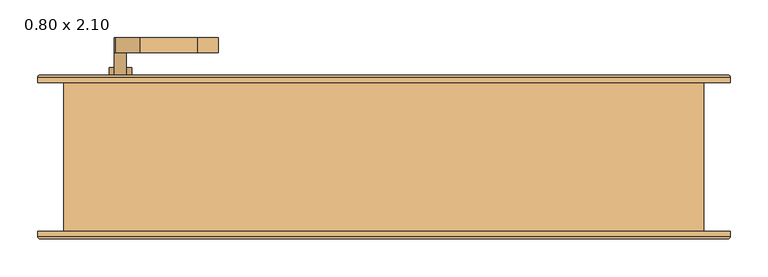
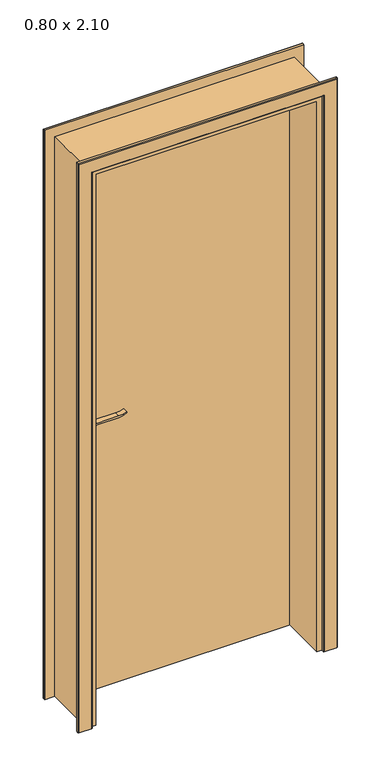
"""IFC4 building model written with IfcOpenShell, lengths in millimetres: door geometry, .CC_ND 300_PORTA SIMPLES DE ABRIR_COM EXTENSÃO : 0.80 x 2.10."""

import ifcopenshell
import ifcopenshell.guid

model = None  # the IFC model being written
_history = None  # IfcOwnerHistory: only IFC2X3 demands one
_inside = {}  # id of a spatial element -> (the spatial element, [elements in it])
_under = {}  # id of a project, library or spatial element -> (it, [spatial elements below it])
_declared = {}  # id of a project -> (the project, [libraries it declares])
_typed = {}  # id of a type object -> (the type object, [elements of that type])
_made_of = {}  # id of a material, layer set ... -> (it, [elements and type objects made of it])


def new_model(schema):
    """Start an empty IFC model of exactly this schema.

    Asked for "IFC4X3", IfcOpenShell would pick the latest addendum, in which some entities
    have other attributes; the version numbers below select the first issue.
    IFC2X3 requires an IfcOwnerHistory on every rooted entity: one is made here for all.
    """
    global model, _history
    if schema == "IFC4X3":
        model = ifcopenshell.file(schema_version=(4, 3, 0, 0))
    else:
        model = ifcopenshell.file(schema=schema)
    _inside.clear()
    _under.clear()
    _declared.clear()
    _typed.clear()
    _made_of.clear()
    _history = None
    if model.schema == "IFC2X3":
        org = make("IfcOrganization", Name="unknown")
        user = make(
            "IfcPersonAndOrganization",
            ThePerson=make("IfcPerson", FamilyName="unknown"),
            TheOrganization=org,
        )
        app = make(
            "IfcApplication",
            ApplicationDeveloper=org,
            Version="unknown",
            ApplicationFullName="unknown",
            ApplicationIdentifier="unknown",
        )
        _history = make(
            "IfcOwnerHistory",
            OwningUser=user,
            OwningApplication=app,
            ChangeAction="ADDED",
            CreationDate=0,
        )
    return model


def make(cls, **values):
    """One entity of the class cls with the attributes given. An attribute that is None is left unset."""
    return model.create_entity(
        cls, **{name: value for name, value in values.items() if value is not None}
    )


def rooted(cls, **values):
    """An entity with a GlobalId (a new one), such as an element, a storey or a relation."""
    return make(cls, GlobalId=ifcopenshell.guid.new(), OwnerHistory=_history, **values)


def si_unit(unit_type, name, prefix=None):
    """IfcSIUnit, for example si_unit("LENGTHUNIT", "METRE", prefix="MILLI")."""
    return make("IfcSIUnit", UnitType=unit_type, Prefix=prefix, Name=name)


def assignment(units):
    """IfcUnitAssignment: the units of a project."""
    return None if units is None else make("IfcUnitAssignment", Units=units)


def point(xyz):
    """IfcCartesianPoint."""
    return None if xyz is None else make("IfcCartesianPoint", Coordinates=xyz)


def direction(xyz):
    """IfcDirection."""
    return None if xyz is None else make("IfcDirection", DirectionRatios=xyz)


def frame(location, z_axis=None, x_axis=None):
    """IfcAxis2Placement3D, a coordinate frame: its origin and axes. An axis left out is left unset."""
    return make(
        "IfcAxis2Placement3D",
        Location=point(location),
        Axis=direction(z_axis),
        RefDirection=direction(x_axis),
    )


def frame_2d(location, x_axis=None):
    """IfcAxis2Placement2D, a coordinate frame in the plane: its origin and x axis."""
    return make(
        "IfcAxis2Placement2D", Location=point(location), RefDirection=direction(x_axis)
    )


def origin():
    """The frame at (0, 0, 0) with its axes left unset."""
    return frame((0.0, 0.0, 0.0))


def origin_with_axes():
    """The frame at (0, 0, 0) with the z axis (0, 0, 1) and the x axis (1, 0, 0) written out."""
    return frame((0.0, 0.0, 0.0), z_axis=(0.0, 0.0, 1.0), x_axis=(1.0, 0.0, 0.0))


def place(relative_to, where):
    """IfcLocalPlacement: puts the frame where relative to a parent placement (None: the world)."""
    return make(
        "IfcLocalPlacement", PlacementRelTo=relative_to, RelativePlacement=where
    )


def context(
    kind, dimensions, precision=None, world=None, true_north=None, identifier=None
):
    """IfcGeometricRepresentationContext, for example the 3D "Model" context."""
    return make(
        "IfcGeometricRepresentationContext",
        ContextIdentifier=identifier,
        ContextType=kind,
        CoordinateSpaceDimension=dimensions,
        Precision=precision,
        WorldCoordinateSystem=world,
        TrueNorth=true_north,
    )


def project(units=None, contexts=None):
    """IfcProject with its units and contexts."""
    return rooted(
        "IfcProject",
        Name="project",
        RepresentationContexts=contexts,
        UnitsInContext=assignment(units),
    )


def spatial(cls, under=None, at=None, **own):
    """A site, building, storey or space (cls), placed at a placement, below another one or the project."""
    s = rooted(cls, ObjectPlacement=at, **own)
    if under is not None:
        _under.setdefault(under.id(), (under, []))[1].append(s)
    return s


def polyline(points):
    """IfcPolyline through the points."""
    return make("IfcPolyline", Points=[point(p) for p in points])


def circle_curve(where, radius):
    """IfcCircle in the frame where."""
    return make("IfcCircle", Position=where, Radius=radius)


def ellipse_curve(where, semi_axis1, semi_axis2):
    """IfcEllipse in the frame where."""
    return make(
        "IfcEllipse", Position=where, SemiAxis1=semi_axis1, SemiAxis2=semi_axis2
    )


def trimmed(basis, trim1, trim2, sense, master):
    """IfcTrimmedCurve: the piece of a basis curve between two trims."""
    return make(
        "IfcTrimmedCurve",
        BasisCurve=basis,
        Trim1=trim1,
        Trim2=trim2,
        SenseAgreement=sense,
        MasterRepresentation=master,
    )


def segment(curve, same_sense, transition):
    """IfcCompositeCurveSegment."""
    return make(
        "IfcCompositeCurveSegment",
        Transition=transition,
        SameSense=same_sense,
        ParentCurve=curve,
    )


def composite_curve(segments, self_intersect=None):
    """IfcCompositeCurve: segments joined end to end."""
    return make("IfcCompositeCurve", Segments=segments, SelfIntersect=self_intersect)


def outline(outer, holes=None, kind="AREA"):
    """IfcArbitraryClosedProfileDef: a profile drawn as a closed curve; with holes, ...WithVoids."""
    if holes is None:
        return make("IfcArbitraryClosedProfileDef", ProfileType=kind, OuterCurve=outer)
    return make(
        "IfcArbitraryProfileDefWithVoids",
        ProfileType=kind,
        OuterCurve=outer,
        InnerCurves=holes,
    )


def extrude(swept, where, along, depth):
    """IfcExtrudedAreaSolid: the profile swept, set in the frame where, extruded along a direction by depth."""
    return make(
        "IfcExtrudedAreaSolid",
        SweptArea=swept,
        Position=where,
        ExtrudedDirection=direction(along),
        Depth=depth,
    )


def faces_of(points, faces, orient=None, outer=None):
    """IfcFace entities. A face is a list of loops; a loop is a list of indices into points, from 0.

    orient and outer hold one flag for each loop. By default every Orientation is true, the
    first loop of a face is its IfcFaceOuterBound and the others are IfcFaceBound.
    """
    made = []
    for i, loops in enumerate(faces):
        bounds = []
        for j, loop in enumerate(loops):
            is_outer = j == 0 if outer is None else outer[i][j]
            bounds.append(
                make(
                    "IfcFaceOuterBound" if is_outer else "IfcFaceBound",
                    Bound=make("IfcPolyLoop", Polygon=[points[k] for k in loop]),
                    Orientation=True if orient is None else orient[i][j],
                )
            )
        made.append(make("IfcFace", Bounds=bounds))
    return made


def faceted_brep(points, faces, orient=None, outer=None, voids=None):
    """IfcFacetedBrep: a solid bounded by flat faces; with voids (closed shells), ...WithVoids."""
    shared = [point(p) for p in points]
    hull = make("IfcClosedShell", CfsFaces=faces_of(shared, faces, orient, outer))
    if voids is None:
        return make("IfcFacetedBrep", Outer=hull)
    return make(
        "IfcFacetedBrepWithVoids",
        Outer=hull,
        Voids=[
            make(cls, CfsFaces=faces_of(shared, fs, o, b)) for cls, fs, o, b in voids
        ],
    )


def shape(context_of_items, identifier, shape_type, items):
    """IfcShapeRepresentation: the items that make up one representation, for example the "Body"."""
    return make(
        "IfcShapeRepresentation",
        ContextOfItems=context_of_items,
        RepresentationIdentifier=identifier,
        RepresentationType=shape_type,
        Items=items,
    )


def source(mapping_origin, context_of_items, identifier, shape_type, items):
    """IfcRepresentationMap: a shape defined once, which mapped items show again and again."""
    return make(
        "IfcRepresentationMap",
        MappingOrigin=mapping_origin,
        MappedRepresentation=shape(context_of_items, identifier, shape_type, items),
    )


def transform(
    local_origin,
    x_axis=None,
    y_axis=None,
    z_axis=None,
    scale=None,
    scale2=None,
    scale3=None,
    uniform=True,
):
    """IfcCartesianTransformationOperator3D, or its non-uniform kind. x_axis, y_axis, z_axis: its Axis1, 2, 3."""
    if uniform:
        return make(
            "IfcCartesianTransformationOperator3D",
            Axis1=direction(x_axis),
            Axis2=direction(y_axis),
            LocalOrigin=point(local_origin),
            Scale=scale,
            Axis3=direction(z_axis),
        )
    return make(
        "IfcCartesianTransformationOperator3DnonUniform",
        Axis1=direction(x_axis),
        Axis2=direction(y_axis),
        LocalOrigin=point(local_origin),
        Scale=scale,
        Axis3=direction(z_axis),
        Scale2=scale2,
        Scale3=scale3,
    )


def mapped(mapping_source, mapping_target):
    """IfcMappedItem: shows the shape of a source again, moved by a transform."""
    return make(
        "IfcMappedItem", MappingSource=mapping_source, MappingTarget=mapping_target
    )


def made_of(thing, what):
    """Note that an element or type object is made of a material, layer set ...; save() writes the relation."""
    if what is not None:
        _made_of.setdefault(what.id(), (what, []))[1].append(thing)
    return thing


def element(
    cls,
    number,
    at=None,
    inside=None,
    cuts=None,
    type_object=None,
    material=None,
    context=None,
    identifier="Body",
    shape_type=None,
    held_by="IfcProductDefinitionShape",
    body=None,
    shapes=None,
    **own,
):
    """One element of the class cls, such as IfcWall. Its Tag is "e" and its number.

    at: its placement. inside: the storey or other place that contains it. cuts: it is an
    opening in that element (IfcRelVoidsElement). A single representation is given by context,
    identifier, shape_type and body (its items); several are given by shapes. held_by: the class
    of the entity that holds the representations. save() writes the other relations.
    """
    e = rooted(cls, Tag="e%d" % number, ObjectPlacement=at, **own)
    if body is not None:
        shapes = [shape(context, identifier, shape_type, body)]
    if shapes is not None:
        e.Representation = make(held_by, Representations=shapes)
    if inside is not None:
        _inside.setdefault(inside.id(), (inside, []))[1].append(e)
    if cuts is not None:
        rooted(
            "IfcRelVoidsElement", RelatingBuildingElement=cuts, RelatedOpeningElement=e
        )
    if type_object is not None:
        _typed.setdefault(type_object.id(), (type_object, []))[1].append(e)
    return made_of(e, material)


def aggregate(whole, parts):
    """IfcRelAggregates: a whole, such as a stair, and the parts it consists of."""
    return rooted("IfcRelAggregates", RelatingObject=whole, RelatedObjects=parts)


def save(model, path):
    """Write the relations noted so far, then the file.

    IfcRelAggregates (storeys below a building ...), IfcRelContainedInSpatialStructure (elements
    in a storey), IfcRelDefinesByType, IfcRelAssociatesMaterial and IfcRelDeclares: one each for
    every whole, place, type object, material and project.
    """
    for whole, parts in _under.values():
        aggregate(whole, parts)
    for where, things in _inside.values():
        rooted(
            "IfcRelContainedInSpatialStructure",
            RelatedElements=things,
            RelatingStructure=where,
        )
    for kind, things in _typed.values():
        rooted("IfcRelDefinesByType", RelatedObjects=things, RelatingType=kind)
    for what, things in _made_of.values():
        rooted("IfcRelAssociatesMaterial", RelatedObjects=things, RelatingMaterial=what)
    for by, libraries in _declared.values():
        rooted("IfcRelDeclares", RelatingContext=by, RelatedDefinitions=libraries)
    model.write(path)


def plane_surface(at):
    """IfcPlane: the flat surface through the origin of the frame at, square to its z axis."""
    return make("IfcPlane", Position=at)


def cylinder_surface(at, radius):
    """IfcCylindricalSurface: all points at the distance radius from the z axis of the frame at."""
    return make("IfcCylindricalSurface", Position=at, Radius=radius)


def advanced_brep(points, edges, surfaces, faces):
    """IfcAdvancedBrep: a solid bounded by faces that lie on surfaces and meet in shared edges.

    An edge is (start, end): straight between two places in points (the first is 0);
    or (start, end, curve); or (start, end, curve, False) where it runs against its curve.
    A face is (place in surfaces, loops), or (place, loops, False) where it looks against
    its surface's normal. A loop lists edges by number (the first is 1), with a minus sign
    where the edge is run from its end to its start. The first loop is the outer one.
    """
    corners = [point(p) for p in points]
    vertices = [make("IfcVertexPoint", VertexGeometry=c) for c in corners]
    made = []
    for start, end, *more in edges:
        made.append(
            make(
                "IfcEdgeCurve",
                EdgeStart=vertices[start],
                EdgeEnd=vertices[end],
                EdgeGeometry=more[0] if more else make("IfcPolyline", Points=[corners[start], corners[end]]),
                SameSense=more[1] if len(more) > 1 else True,
            )
        )
    hull = []
    for where, loops, *sense in faces:
        bounds = []
        for j, loop in enumerate(loops):
            ring = [make("IfcOrientedEdge", EdgeElement=made[abs(k) - 1], Orientation=k > 0) for k in loop]
            bounds.append(
                make(
                    "IfcFaceOuterBound" if j == 0 else "IfcFaceBound",
                    Bound=make("IfcEdgeLoop", EdgeList=ring),
                    Orientation=True,
                )
            )
        hull.append(make("IfcAdvancedFace", Bounds=bounds, FaceSurface=surfaces[where], SameSense=sense[0] if sense else True))
    return make("IfcAdvancedBrep", Outer=make("IfcClosedShell", CfsFaces=hull))


def door_0_80_x_2_10_6188e507(model_context):
    return source(origin(), model_context, "Body", "SolidModel", [
        extrude(outline(composite_curve([segment(trimmed(circle_curve(frame_2d((964.5, -350.0)), 15.0), [point((964.5, -335.0))], [point((964.5, -365.0))], False, "CARTESIAN"), True, "CONTINUOUS"), segment(trimmed(circle_curve(frame_2d((964.5, -350.0)), 15.0), [point((964.5, -365.0))], [point((964.5, -335.0))], False, "CARTESIAN"), True, "CONTINUOUS")], self_intersect=False)), frame((0.0, 108.8, 0.0), z_axis=(0.0, 1.0, 0.0), x_axis=(0.0, 0.0, 1.0)), (0.0, 0.0, 1.0), 10.0),
        extrude(outline(composite_curve([segment(trimmed(circle_curve(frame_2d((964.5, -350.0)), 15.0), [point((964.5, -335.0))], [point((964.5, -365.0))], False, "CARTESIAN"), True, "CONTINUOUS"), segment(trimmed(circle_curve(frame_2d((964.5, -350.0)), 15.0), [point((964.5, -365.0))], [point((964.5, -335.0))], False, "CARTESIAN"), True, "CONTINUOUS")], self_intersect=False)), frame((0.0, 48.8, 0.0), z_axis=(0.0, 1.0, 0.0), x_axis=(0.0, 0.0, 1.0)), (0.0, 0.0, 1.0), 10.0),
        extrude(outline(composite_curve([segment(trimmed(circle_curve(frame_2d((1024.5, -350.0)), 8.0), [point((1029.1523287, -356.5081363))], [point((1024.5, -342.0))], False, "CARTESIAN"), True, "CONTINUOUS"), segment(trimmed(circle_curve(frame_2d((1019.3738613, -324.6138099)), 18.1261387), [point((1024.5, -342.0))], [point((1037.5, -324.6138099))], True, "CARTESIAN"), True, "CONTINUOUS"), segment(polyline([(1037.5, -324.6138099), (1037.5, -248.3564091)]), True, "CONTINUOUS"), segment(trimmed(circle_curve(frame_2d((1096.7709207, -251.9396612)), 59.3791355), [point((1037.5, -248.3564091))], [point((1046.7135558, -220.0))], False, "CARTESIAN"), True, "CONTINUOUS"), segment(polyline([(1046.7135558, -220.0), (1049.5, -220.0)]), True, "CONTINUOUS"), segment(trimmed(circle_curve(frame_2d((1127.7850638, -248.4227909)), 83.2850902), [point((1049.5, -220.0))], [point((1044.5, -248.3564091))], True, "CARTESIAN"), True, "CONTINUOUS"), segment(polyline([(1044.5, -248.3564091), (1044.5, -324.6325667)]), True, "CONTINUOUS"), segment(trimmed(circle_curve(frame_2d((1007.2555521, -326.3324871)), 37.2832219), [point((1044.5, -324.6325667))], [point((1029.1523287, -356.5081363))], False, "CARTESIAN"), True, "CONTINUOUS")], self_intersect=False)), frame((0.0, 138.8, 0.0), z_axis=(0.0, 1.0, 0.0), x_axis=(0.0, 0.0, 1.0)), (0.0, 0.0, 1.0), 20.0),
        extrude(outline(composite_curve([segment(trimmed(circle_curve(frame_2d((1019.3738682, -324.6138122)), 18.1261318), [point((1024.4999903, -342.0))], [point((1037.5, -324.6138122))], True, "CARTESIAN"), True, "CONTINUOUS"), segment(polyline([(1037.5, -324.6138122), (1037.5, -248.3564091)]), True, "CONTINUOUS"), segment(trimmed(circle_curve(frame_2d((1096.7709207, -251.9396612)), 59.3791355), [point((1037.5, -248.3564091))], [point((1046.7135558, -220.0))], False, "CARTESIAN"), True, "CONTINUOUS"), segment(polyline([(1046.7135558, -220.0), (1049.5, -220.0)]), True, "CONTINUOUS"), segment(trimmed(circle_curve(frame_2d((1127.7850638, -248.4227909)), 83.2850902), [point((1049.5, -220.0))], [point((1044.5, -248.3564091))], True, "CARTESIAN"), True, "CONTINUOUS"), segment(polyline([(1044.5, -248.3564091), (1044.5, -324.6325667)]), True, "CONTINUOUS"), segment(trimmed(circle_curve(frame_2d((1007.2555521, -326.3324871)), 37.2832219), [point((1044.5, -324.6325667))], [point((1029.1523287, -356.5081363))], False, "CARTESIAN"), True, "CONTINUOUS"), segment(trimmed(circle_curve(frame_2d((1024.5, -350.0)), 8.0), [point((1029.1523287, -356.5081363))], [point((1024.4999903, -342.0))], False, "CARTESIAN"), True, "CONTINUOUS")], self_intersect=False)), frame((0.0, 8.8, 0.0), z_axis=(0.0, 1.0, 0.0), x_axis=(0.0, 0.0, 1.0)), (0.0, 0.0, 1.0), 20.0),
        extrude(outline(composite_curve([segment(trimmed(circle_curve(frame_2d((1024.5, -350.0)), 8.0), [point((1024.5, -342.0))], [point((1024.5, -358.0))], False, "CARTESIAN"), True, "CONTINUOUS"), segment(trimmed(circle_curve(frame_2d((1024.5, -350.0)), 8.0), [point((1024.5, -358.0))], [point((1024.5, -342.0))], False, "CARTESIAN"), True, "CONTINUOUS")], self_intersect=False)), frame((0.0, 108.8, 0.0), z_axis=(0.0, 1.0, 0.0), x_axis=(0.0, 0.0, 1.0)), (0.0, 0.0, 1.0), 30.0),
        extrude(outline(composite_curve([segment(trimmed(circle_curve(frame_2d((1024.5, -350.0)), 8.0), [point((1024.5, -342.0))], [point((1024.5, -358.0))], False, "CARTESIAN"), True, "CONTINUOUS"), segment(trimmed(circle_curve(frame_2d((1024.5, -350.0)), 8.0), [point((1024.5, -358.0))], [point((1024.5, -342.0))], False, "CARTESIAN"), True, "CONTINUOUS")], self_intersect=False)), frame((0.0, 28.8, 0.0), z_axis=(0.0, 1.0, 0.0), x_axis=(0.0, 0.0, 1.0)), (0.0, 0.0, 1.0), 30.0),
        extrude(outline(composite_curve([segment(trimmed(circle_curve(frame_2d((954.5, -350.0)), 25.0), [point((954.5, -375.0))], [point((954.5, -325.0))], False, "CARTESIAN"), True, "CONTINUOUS"), segment(polyline([(954.5, -325.0), (1024.5, -325.0)]), True, "CONTINUOUS"), segment(trimmed(circle_curve(frame_2d((1024.5, -350.0)), 25.0), [point((1024.5, -325.0))], [point((1024.5, -375.0))], False, "CARTESIAN"), True, "CONTINUOUS"), segment(polyline([(1024.5, -375.0), (954.5, -375.0)]), True, "CONTINUOUS")], self_intersect=False)), frame((0.0, 98.8, 0.0), z_axis=(0.0, 1.0, 0.0), x_axis=(0.0, 0.0, 1.0)), (0.0, 0.0, 1.0), 10.0),
        extrude(outline(composite_curve([segment(trimmed(circle_curve(frame_2d((954.5, -350.0)), 25.0), [point((954.5, -375.0))], [point((954.5, -325.0))], False, "CARTESIAN"), True, "CONTINUOUS"), segment(polyline([(954.5, -325.0), (1024.5, -325.0)]), True, "CONTINUOUS"), segment(trimmed(circle_curve(frame_2d((1024.5, -350.0)), 25.0), [point((1024.5, -325.0))], [point((1024.5, -375.0))], False, "CARTESIAN"), True, "CONTINUOUS"), segment(polyline([(1024.5, -375.0), (954.5, -375.0)]), True, "CONTINUOUS")], self_intersect=False)), frame((0.0, 58.8, 0.0), z_axis=(0.0, 1.0, 0.0), x_axis=(0.0, 0.0, 1.0)), (0.0, 0.0, 1.0), 10.0),
        advanced_brep(
        [(-460.0, 98.8, 0.0), (-460.0, 105.8, 0.0), (-457.0, 108.8, 0.0), (-413.0, 108.8, 0.0), (-410.0, 105.8, 0.0), (-410.0, 98.8, 0.0), (-410.0, 98.8, 2085.0), (410.0, 98.8, 2085.0), (410.0, 98.8, 0.0), (460.0, 98.8, 0.0), (460.0, 98.8, 2135.0), (-460.0, 98.8, 2135.0), (-410.0, 105.8, 2085.0), (-413.0, 108.8, 2088.0), (-457.0, 108.8, 2132.0), (457.0, 108.8, 2132.0), (457.0, 108.8, 0.0), (413.0, 108.8, 0.0), (413.0, 108.8, 2088.0), (-460.0, 105.8, 2135.0), (460.0, 105.8, 0.0), (460.0, 105.8, 2135.0), (410.0, 105.8, 0.0), (410.0, 105.8, 2085.0)],
        [
            (0, 1),
            (1, 2, circle_curve(frame((-457.0, 105.8, 0.0), z_axis=(0.0, 0.0, -1.0), x_axis=(1.0, 0.0, 0.0)), 3.0)),
            (2, 3),
            (3, 4, circle_curve(frame((-413.0, 105.8, 0.0), z_axis=(0.0, 0.0, -1.0), x_axis=(1.0, 0.0, 0.0)), 3.0)),
            (4, 5),
            (5, 0),
            (5, 6),
            (6, 7),
            (7, 8),
            (8, 9),
            (9, 10),
            (10, 11),
            (11, 0),
            (4, 12),
            (12, 6),
            (3, 13),
            (13, 12, ellipse_curve(frame((-413.0, 105.8, 2088.0), z_axis=(-0.7071067811865475, 0.0, -0.7071067811865475), x_axis=(0.7071067811865474, 0.0, -0.7071067811865476)), 4.2426407, 3.0)),
            (2, 14),
            (14, 15),
            (15, 16),
            (16, 17),
            (17, 18),
            (18, 13),
            (1, 19),
            (19, 14, ellipse_curve(frame((-457.0, 105.8, 2132.0), z_axis=(-0.7071067811865475, 0.0, -0.7071067811865475), x_axis=(0.7071067811865474, 0.0, -0.7071067811865476)), 4.2426407, 3.0)),
            (11, 19),
            (9, 20),
            (20, 21),
            (21, 10),
            (8, 22),
            (22, 17, circle_curve(frame((413.0, 105.8, 0.0), z_axis=(0.0, 0.0, -1.0), x_axis=(-1.0, 0.0, 0.0)), 3.0)),
            (16, 20, circle_curve(frame((457.0, 105.8, 0.0), z_axis=(0.0, 0.0, -1.0), x_axis=(-1.0, 0.0, 0.0)), 3.0)),
            (23, 22),
            (7, 23),
            (23, 18, ellipse_curve(frame((413.0, 105.8, 2088.0), z_axis=(0.7071067811865475, 0.0, -0.7071067811865475), x_axis=(0.7071067811865474, 0.0, 0.7071067811865476)), 4.2426407, 3.0)),
            (15, 21, ellipse_curve(frame((457.0, 105.8, 2132.0), z_axis=(0.7071067811865475, 0.0, -0.7071067811865475), x_axis=(0.7071067811865474, 0.0, 0.7071067811865476)), 4.2426407, 3.0)),
            (12, 23),
            (21, 19),
        ],
        [
            plane_surface(frame((-410.0, 98.8, 0.0), z_axis=(0.0, 0.0, -1.0), x_axis=(0.0, -1.0, 0.0))),
            plane_surface(frame((-460.0, 98.8, 0.0), z_axis=(0.0, -1.0, 0.0), x_axis=(0.0, 0.0, 1.0))),
            plane_surface(frame((-410.0, 98.8, 0.0), z_axis=(1.0, 0.0, 0.0), x_axis=(0.0, 0.0, 1.0))),
            cylinder_surface(frame((-413.0, 105.8, 0.0), z_axis=(0.0, 0.0, -1.0), x_axis=(1.0, 0.0, 0.0)), 3.0),
            plane_surface(frame((-413.0, 108.8, 0.0), z_axis=(0.0, 1.0, 0.0), x_axis=(0.0, 0.0, 1.0))),
            cylinder_surface(frame((-457.0, 105.8, 0.0), z_axis=(0.0, 0.0, -1.0), x_axis=(1.0, 0.0, 0.0)), 3.0),
            plane_surface(frame((-460.0, 105.8, 0.0), z_axis=(-1.0, 0.0, 0.0), x_axis=(0.0, 0.0, 1.0))),
            plane_surface(frame((460.0, 105.8, 2135.0), z_axis=(1.0, 0.0, 0.0), x_axis=(0.0, 0.0, -1.0))),
            plane_surface(frame((410.0, 98.8, 0.0), z_axis=(0.0, 0.0, -1.0), x_axis=(0.0, -1.0, 0.0))),
            plane_surface(frame((410.0, 98.8, 2085.0), z_axis=(-1.0, 0.0, 0.0), x_axis=(0.0, 0.0, -1.0))),
            cylinder_surface(frame((413.0, 105.8, 2085.0), z_axis=(0.0, 0.0, 1.0), x_axis=(-1.0, 0.0, 0.0)), 3.0),
            cylinder_surface(frame((457.0, 105.8, 2085.0), z_axis=(0.0, 0.0, 1.0), x_axis=(-1.0, 0.0, 0.0)), 3.0),
            plane_surface(frame((-410.0, 98.8, 2085.0), z_axis=(0.0, 0.0, -1.0), x_axis=(1.0, 0.0, 0.0))),
            plane_surface(frame((-460.0, 105.8, 2135.0), z_axis=(0.0, 0.0, 1.0), x_axis=(1.0, 0.0, 0.0))),
            cylinder_surface(frame((-410.0, 105.8, 2088.0), z_axis=(-1.0, 0.0, 0.0), x_axis=(0.0, 0.0, -1.0)), 3.0),
            cylinder_surface(frame((-410.0, 105.8, 2132.0), z_axis=(-1.0, 0.0, 0.0), x_axis=(0.0, 0.0, -1.0)), 3.0),
        ],
        [
            (0, [[1, 2, 3, 4, 5, 6]]),
            (1, [[7, 8, 9, 10, 11, 12, 13, -6]]),
            (2, [[14, 15, -7, -5]]),
            (3, [[16, 17, -14, -4]]),
            (4, [[18, 19, 20, 21, 22, 23, -16, -3]]),
            (5, [[24, 25, -18, -2]]),
            (6, [[-13, 26, -24, -1]]),
            (7, [[-11, 27, 28, 29]]),
            (8, [[-10, 30, 31, -21, 32, -27]]),
            (9, [[33, -30, -9, 34]]),
            (10, [[-22, -31, -33, 35]]),
            (11, [[-28, -32, -20, 36]]),
            (12, [[37, -34, -8, -15]]),
            (13, [[-12, -29, 38, -26]]),
            (14, [[-23, -35, -37, -17]]),
            (15, [[-38, -36, -19, -25]]),
        ],
    ),
        advanced_brep(
        [(460.0, -98.8, 0.0), (460.0, -105.8342217, 0.0), (457.0342217, -108.8, 0.0), (412.9842717, -108.8, 0.0), (410.0, -105.8157283, 0.0), (410.0, -98.8, 0.0), (410.0, -98.8, 2085.0), (-410.0, -98.8, 2085.0), (-410.0, -98.8, 0.0), (-460.0, -98.8, 0.0), (-460.0, -98.8, 2135.0), (460.0, -98.8, 2135.0), (410.0, -105.8157283, 2085.0), (412.9842717, -108.8, 2087.9842717), (457.0342217, -108.8, 2132.0342217), (-457.0342217, -108.8, 2132.0342217), (-457.0342217, -108.8, 0.0), (-412.9842717, -108.8, 0.0), (-412.9842717, -108.8, 2087.9842717), (460.0, -105.8342217, 2135.0), (-460.0, -105.8342217, 0.0), (-460.0, -105.8342217, 2135.0), (-410.0, -105.8157283, 0.0), (-410.0, -105.8157283, 2085.0)],
        [
            (0, 1),
            (1, 2, circle_curve(frame((457.0342217, -105.8342217, 0.0), z_axis=(0.0, 0.0, -1.0), x_axis=(1.0, 0.0, 0.0)), 2.9657783)),
            (2, 3),
            (3, 4, circle_curve(frame((412.9842717, -105.8157283, 0.0), z_axis=(0.0, 0.0, -1.0), x_axis=(1.0, 0.0, 0.0)), 2.9842717)),
            (4, 5),
            (5, 0),
            (5, 6),
            (6, 7),
            (7, 8),
            (8, 9),
            (9, 10),
            (10, 11),
            (11, 0),
            (4, 12),
            (12, 6),
            (3, 13),
            (13, 12, ellipse_curve(frame((412.9842717, -105.8157283, 2087.9842717), z_axis=(0.7071067811865475, 0.0, -0.7071067811865475), x_axis=(-0.7071067811865474, 0.0, -0.7071067811865476)), 4.2203975, 2.9842717)),
            (2, 14),
            (14, 15),
            (15, 16),
            (16, 17),
            (17, 18),
            (18, 13),
            (1, 19),
            (19, 14, ellipse_curve(frame((457.0342217, -105.8342217, 2132.0342217), z_axis=(0.7071067811865475, 0.0, -0.7071067811865475), x_axis=(-0.7071067811865474, 0.0, -0.7071067811865476)), 4.1942438, 2.9657783)),
            (11, 19),
            (9, 20),
            (20, 21),
            (21, 10),
            (8, 22),
            (22, 17, circle_curve(frame((-412.9842717, -105.8157283, 0.0), z_axis=(0.0, 0.0, -1.0), x_axis=(-1.0, 0.0, 0.0)), 2.9842717)),
            (16, 20, circle_curve(frame((-457.0342217, -105.8342217, 0.0), z_axis=(0.0, 0.0, -1.0), x_axis=(-1.0, 0.0, 0.0)), 2.9657783)),
            (23, 22),
            (7, 23),
            (23, 18, ellipse_curve(frame((-412.9842717, -105.8157283, 2087.9842717), z_axis=(-0.7071067811865475, 0.0, -0.7071067811865475), x_axis=(-0.7071067811865474, 0.0, 0.7071067811865476)), 4.2203975, 2.9842717)),
            (15, 21, ellipse_curve(frame((-457.0342217, -105.8342217, 2132.0342217), z_axis=(-0.7071067811865475, 0.0, -0.7071067811865475), x_axis=(-0.7071067811865474, 0.0, 0.7071067811865476)), 4.1942438, 2.9657783)),
            (12, 23),
            (21, 19),
        ],
        [
            plane_surface(frame((410.0, -98.8, 0.0), z_axis=(0.0, 0.0, -1.0), x_axis=(0.0, -1.0, 0.0))),
            plane_surface(frame((460.0, -98.8, 0.0), z_axis=(0.0, 1.0, 0.0), x_axis=(0.0, 0.0, 1.0))),
            plane_surface(frame((410.0, -98.8, 0.0), z_axis=(-1.0, 0.0, 0.0), x_axis=(0.0, 0.0, 1.0))),
            cylinder_surface(frame((412.9842717, -105.8157283, 0.0), z_axis=(0.0, 0.0, -1.0), x_axis=(1.0, 0.0, 0.0)), 2.9842717),
            plane_surface(frame((412.9842717, -108.8, 0.0), z_axis=(0.0, -1.0, 0.0), x_axis=(0.0, 0.0, 1.0))),
            cylinder_surface(frame((457.0342217, -105.8342217, 0.0), z_axis=(0.0, 0.0, -1.0), x_axis=(1.0, 0.0, 0.0)), 2.9657783),
            plane_surface(frame((460.0, -105.8342217, 0.0), z_axis=(1.0, 0.0, 0.0), x_axis=(0.0, 0.0, 1.0))),
            plane_surface(frame((-460.0, -105.8342217, 2135.0), z_axis=(-1.0, 0.0, 0.0), x_axis=(0.0, 0.0, -1.0))),
            plane_surface(frame((-410.0, -98.8, 0.0), z_axis=(0.0, 0.0, -1.0), x_axis=(0.0, -1.0, 0.0))),
            plane_surface(frame((-410.0, -98.8, 2085.0), z_axis=(1.0, 0.0, 0.0), x_axis=(0.0, 0.0, -1.0))),
            cylinder_surface(frame((-412.9842717, -105.8157283, 2085.0), z_axis=(0.0, 0.0, 1.0), x_axis=(-1.0, 0.0, 0.0)), 2.9842717),
            cylinder_surface(frame((-457.0342217, -105.8342217, 2085.0), z_axis=(0.0, 0.0, 1.0), x_axis=(-1.0, 0.0, 0.0)), 2.9657783),
            plane_surface(frame((410.0, -98.8, 2085.0), z_axis=(0.0, 0.0, -1.0), x_axis=(-1.0, 0.0, 0.0))),
            plane_surface(frame((460.0, -105.8342217, 2135.0), z_axis=(0.0, 0.0, 1.0), x_axis=(-1.0, 0.0, 0.0))),
            cylinder_surface(frame((410.0, -105.8157283, 2087.9842717), z_axis=(1.0, 0.0, 0.0), x_axis=(0.0, 0.0, 1.0)), 2.9842717),
            cylinder_surface(frame((410.0, -105.8342217, 2132.0342217), z_axis=(1.0, 0.0, 0.0), x_axis=(0.0, 0.0, 1.0)), 2.9657783),
        ],
        [
            (0, [[1, 2, 3, 4, 5, 6]]),
            (1, [[7, 8, 9, 10, 11, 12, 13, -6]]),
            (2, [[14, 15, -7, -5]]),
            (3, [[16, 17, -14, -4]]),
            (4, [[18, 19, 20, 21, 22, 23, -16, -3]]),
            (5, [[24, 25, -18, -2]]),
            (6, [[-13, 26, -24, -1]]),
            (7, [[-11, 27, 28, 29]]),
            (8, [[-10, 30, 31, -21, 32, -27]]),
            (9, [[33, -30, -9, 34]]),
            (10, [[-22, -31, -33, 35]]),
            (11, [[-28, -32, -20, 36]]),
            (12, [[37, -34, -8, -15]]),
            (13, [[-12, -29, 38, -26]]),
            (14, [[-23, -35, -37, -17]]),
            (15, [[-38, -36, -19, -25]]),
        ],
    ),
        faceted_brep([(392.0, -98.8, 0.0), (392.0, 68.8, 0.0), (400.0, 68.8, 0.0), (400.0, 98.8, 0.0), (425.0, 98.8, 0.0), (425.0, -98.8, 0.0), (425.0, -98.8, 2100.0), (-425.0, -98.8, 2100.0), (-425.0, -98.8, 0.0), (-392.0, -98.8, 0.0), (-392.0, -98.8, 2067.0), (392.0, -98.8, 2067.0), (425.0, 98.8, 2100.0), (400.0, 98.8, 2075.0), (-400.0, 98.8, 2075.0), (-400.0, 98.8, 0.0), (-425.0, 98.8, 0.0), (-425.0, 98.8, 2100.0), (400.0, 68.8, 2075.0), (392.0, 68.8, 2067.0), (-392.0, 68.8, 2067.0), (-392.0, 68.8, 0.0), (-400.0, 68.8, 0.0), (-400.0, 68.8, 2075.0)], [[[0, 1, 2, 3, 4, 5]], [[5, 6, 7, 8, 9, 10, 11, 0]], [[4, 12, 6, 5]], [[3, 13, 14, 15, 16, 17, 12, 4]], [[2, 18, 13, 3]], [[1, 19, 20, 21, 22, 23, 18, 2]], [[0, 11, 19, 1]], [[10, 9, 21, 20]], [[9, 8, 16, 15, 22, 21]], [[17, 16, 8, 7]], [[23, 22, 15, 14]], [[12, 17, 7, 6]], [[18, 23, 14, 13]], [[11, 10, 20, 19]]]),
        extrude(outline(polyline([(-400.0, 68.8), (-400.0, 98.8), (400.0, 98.8), (400.0, 68.8), (-400.0, 68.8)])), origin_with_axes(), (0.0, 0.0, 1.0), 2075.0),
    ])


if __name__ == "__main__":
    model = new_model("IFC4")
    model_context = context("Model", 3, world=origin())
    ifc_project = project(units=[si_unit("LENGTHUNIT", "METRE", prefix="MILLI")], contexts=[model_context])
    site = spatial("IfcSite", under=ifc_project)
    building = spatial("IfcBuilding", under=site)
    placement = place(None, origin())
    door_0_80_x_2_10_shape = door_0_80_x_2_10_6188e507(model_context)
    element("IfcDoor", 1, ObjectType=".CC_ND 300_PORTA SIMPLES DE ABRIR_COM EXTENSÃO : 0.80 x 2.10", at=placement, inside=building, context=model_context, shape_type="MappedRepresentation", body=[
        mapped(door_0_80_x_2_10_shape, transform((0.0, 0.0, 0.0), x_axis=(1.0, 0.0, 0.0), y_axis=(0.0, 1.0, 0.0), z_axis=(0.0, 0.0, 1.0))),
    ])
    save(model, "model.ifc")

# Revit data of these elements
# Type ".CC_ND 300_PORTA SIMPLES DE ABRIR_COM EXTENSÃO : 0.80 x 2.10"
#   Type Mark = "153"
#   Rough Width = 0.85 m
#   Espessura moldura externa = 0.01 m
#   Espessura moldura interna = 0.01 m
#   Largura moldura = 0.05 m
#   Extensão acabamento exterior [instance default] = 0.00 m
#   Extensão acabamento interior [instance default] = 0.00 m
#   Espessura batente = 0.025 m
#   Thickness = 0.03 m
#   Altura batente = 2.085 m
#   Aux Arco [instance default] = 0.80 m
#   Rough Height = 2.125 m
#   Height = 2.10 m
#   Width = 0.80 m
#   Moldura interna [instance default] = yes
#   Moldura externa [instance default] = yes
#   Porta = .MADEIRA COM PINTURA ESMALTE BRANCO ACETINADO
#   Moldura = .MADEIRA COM PINTURA ESMALTE BRANCO ACETINADO
#   Maçaneta = .ALUMÍNIO
#   Batente = .MADEIRA COM PINTURA ESMALTE BRANCO ACETINADO
#   Function = (empty or 0)
#   Wall Closure = (empty or 0)
# Element 1 (IfcDoor, ".CC_ND 300_PORTA SIMPLES DE ABRIR_COM EXTENSÃO : 0.80 x 2.10")
#   Materials on its faces: ".MADEIRA COM PINTURA ESMALTE BRANCO ACETINADO", ".ALUMÍNIO"
# Materials
#   ".MADEIRA COM PINTURA ESMALTE BRANCO ACETINADO": class ".CC_MADEIRAS", colour RGB 240 240 240, transparency 0, Description = "Madeira com pintura esmalte branco acetinado.", Cost = 0
#   ".ALUMÍNIO": class "CC_METAIS", colour RGB 244 244 244, transparency 0, Description = "Material alumínio", Cost = 0
